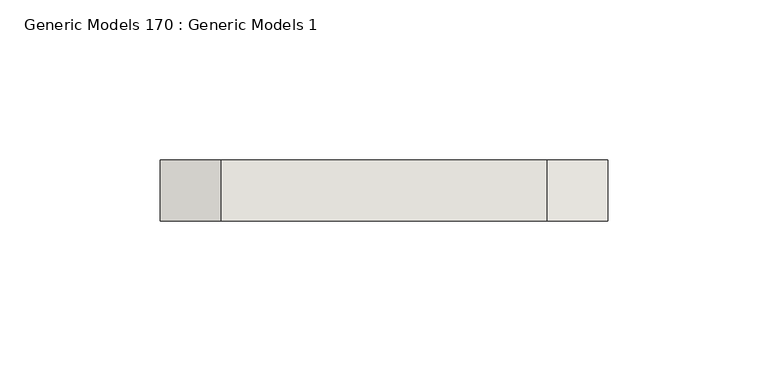
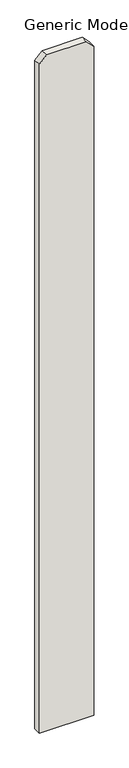
"""IFC4 building model written with IfcOpenShell, lengths in millimetres: wall geometry, Generic Models 170 : Generic Models 1."""

from ifc_helpers import new_model, si_unit, frame, origin, place, context, project, spatial, polyline, outline, extrude, source, transform, mapped, element, save


def generic_models_170_generic_models_1_f7a4aa87(model_context):
    return source(origin(), model_context, "Body", "SweptSolid", [
        extrude(outline(polyline([(76.2, 324889.8125), (1885.95, 324889.8125), (1905.0, 324870.7625), (1905.0, 324769.1625), (1885.95, 324750.1125), (76.2, 324750.1125), (76.2, 324889.8125)])), frame((0.0, 547.6875, 0.0), z_axis=(0.0, 1.0, 0.0), x_axis=(0.0, 0.0, 1.0)), (0.0, 0.0, 1.0), 19.05),
    ])


if __name__ == "__main__":
    model = new_model("IFC4")
    model_context = context("Model", 3, world=origin())
    ifc_project = project(units=[si_unit("LENGTHUNIT", "METRE", prefix="MILLI")], contexts=[model_context])
    site = spatial("IfcSite", under=ifc_project)
    building = spatial("IfcBuilding", under=site)
    placement = place(None, origin())
    generic_models_170_generic_models_1_shape = generic_models_170_generic_models_1_f7a4aa87(model_context)
    element("IfcWall", 1, ObjectType="Generic Models 170 : Generic Models 1", at=placement, inside=building, context=model_context, shape_type="MappedRepresentation", body=[
        mapped(generic_models_170_generic_models_1_shape, transform((0.0, 0.0, 0.0), x_axis=(1.0, 0.0, 0.0), y_axis=(0.0, 1.0, 0.0), z_axis=(0.0, 0.0, 1.0))),
    ])
    save(model, "model.ifc")

# Revit data of these elements
# Element 1 (IfcWall, "Generic Models 170 : Generic Models 1")
#   Materials on its faces: "VERTICAL 1X6 CEDAR PLANKS W/ CLEAR WOOD SEALER"
# Materials
#   "VERTICAL 1X6 CEDAR PLANKS W/ CLEAR WOOD SEALER": class "Wood", colour RGB 234 198 147, transparency 0, Description = "Pinus Echinata", Cost = 0
